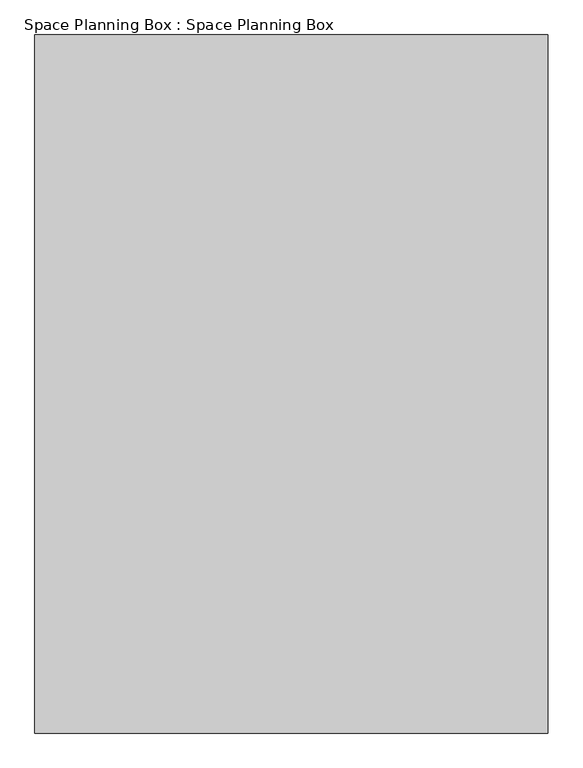
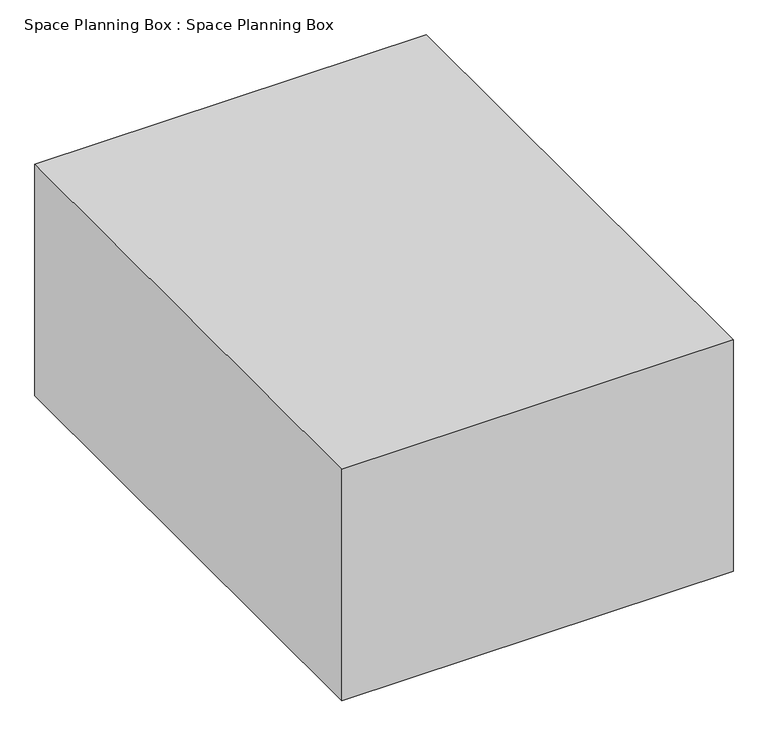
"""IFC4 building model written with IfcOpenShell, lengths in millimetres: proxy geometry, Space Planning Box : Space Planning Box."""

from ifc_helpers import new_model, si_unit, origin, origin_with_axes, place, context, project, spatial, polyline, outline, extrude, source, transform, mapped, element, save


def space_planning_box_space_planning_box_c2e9f8fb(model_context):
    return source(origin(), model_context, "Body", "SweptSolid", [
        extrude(outline(polyline([(4800.0, 6525.0), (4800.0, -6525.0), (-4800.0, -6525.0), (-4800.0, 6525.0), (4800.0, 6525.0)])), origin_with_axes(), (0.0, 0.0, 1.0), 6000.0),
    ])


if __name__ == "__main__":
    model = new_model("IFC4")
    model_context = context("Model", 3, world=origin())
    ifc_project = project(units=[si_unit("LENGTHUNIT", "METRE", prefix="MILLI")], contexts=[model_context])
    site = spatial("IfcSite", under=ifc_project)
    building = spatial("IfcBuilding", under=site)
    placement = place(None, origin())
    space_planning_box_space_planning_box_shape = space_planning_box_space_planning_box_c2e9f8fb(model_context)
    element("IfcBuildingElementProxy", 1, Name="Space Planning Box : Space Planning Box", ObjectType="Space Planning Box : Space Planning Box", at=placement, inside=building, context=model_context, shape_type="MappedRepresentation", body=[
        mapped(space_planning_box_space_planning_box_shape, transform((0.0, 0.0, 0.0), x_axis=(1.0, 0.0, 0.0), y_axis=(0.0, 1.0, 0.0), z_axis=(0.0, 0.0, 1.0))),
    ])
    save(model, "model.ifc")

# Revit data of these elements
# Type "Space Planning Box : Space Planning Box"
#   Type Comments = "..."
#   Room Name [instance default] = "?"
#   Assembly Code = "..."
#   Width [instance default] = 1524 mm
#   Program Area [instance default] = 0 m²
#   Length [instance default] = 1524 mm
#   Height [instance default] = 1524 mm
#   Area [instance default] = 2.32258 m²
#   Fill Color [instance default] = Cyan
#   Default Elevation = 0
# Element 1 (IfcBuildingElementProxy, "Space Planning Box : Space Planning Box")
#   Room Name = "Engineer Room"
#   Width = 9600 mm
#   Program Area = 120 m²
#   Length = 13050 mm
#   Height = 6000 mm
#   Area = 125.28 m²
#   Fill Color = Lime
#   Materials on its faces: "Lime"
# Materials
#   "Cyan": class "Generic", colour RGB 0 255 255, transparency 0.2, Cost = 0
#   "Lime": class "Generic", colour RGB 0 255 0, transparency 0.2, Cost = 0
